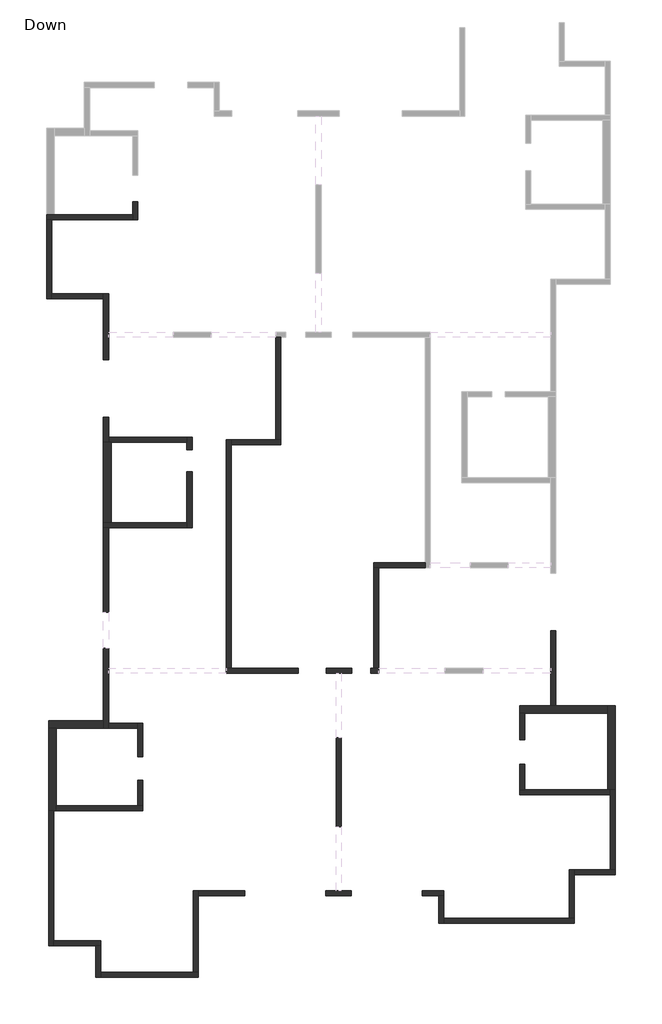
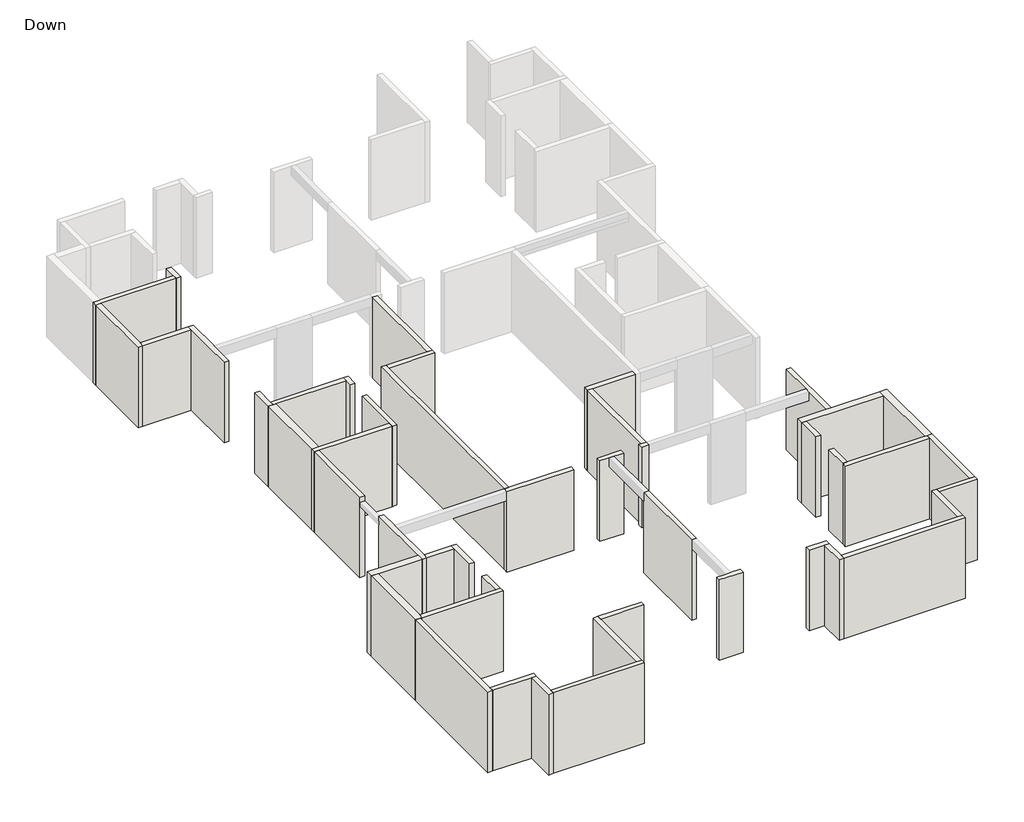
# One storey, part 1 of 2: 47 walls.
"""IFC4 building model written with IfcOpenShell, lengths in millimetres."""

from ifc_helpers import new_model, si_unit, origin, place, context, project, spatial, faceted_brep, element, save

model = new_model("IFC4")

# Units and contexts
model_context = context("Model", 3, world=origin())
ifc_project = project(units=[si_unit("LENGTHUNIT", "METRE", prefix="MILLI")], contexts=[model_context])

# Site, building, storey
site = spatial("IfcSite", under=ifc_project)
building = spatial("IfcBuilding", under=site)
storey = spatial("IfcBuildingStorey", under=building, Name="Down", Elevation=0.0)

# Walls
placement = place(None, origin())
element("IfcWall", 1, ObjectType="20", at=placement, inside=storey, context=model_context, shape_type="Brep", body=[
    faceted_brep([(-11352.0616697, 15349.6557961, 0.0), (-11352.0616697, 14832.6787416, 0.0), (-11352.0616697, 14632.6787416, 0.0), (-11352.0616697, 14632.6787416, 3600.0), (-11352.0616697, 14832.6787416, 3600.0), (-11352.0616697, 15349.6557961, 3600.0), (-11352.0616697, 15349.6557961, 3360.0), (-11152.0616697, 15349.6557961, 0.0), (-11152.0616697, 15349.6557961, 3360.0), (-11152.0616697, 15349.6557961, 3600.0), (-11152.0616697, 14632.6787416, 3600.0), (-11152.0616697, 14632.6787416, 3360.0), (-11152.0616697, 14632.6787416, 0.0)], [[[0, 1, 2, 3, 4, 5, 6]], [[7, 8, 9, 10, 11, 12]], [[2, 1, 0, 7, 12]], [[5, 4, 3, 10, 9]], [[0, 6, 5, 9, 8, 7]], [[3, 2, 12, 11, 10]]]),
])
element("IfcWall", 2, ObjectType="20", at=placement, inside=storey, context=model_context, shape_type="Brep", body=[
    faceted_brep([(-11352.0616697, 14832.6787416, 0.0), (-14451.9956956, 14832.6787416, 0.0), (-14752.0616697, 14832.6787416, 0.0), (-14752.0616697, 14832.6787416, 3600.0), (-14451.9956956, 14832.6787416, 3600.0), (-11352.0616697, 14832.6787416, 3600.0), (-11352.0616697, 14832.6787416, 3360.0), (-11352.0616697, 14632.6787416, 0.0), (-11352.0616697, 14632.6787416, 3600.0), (-14552.0616697, 14632.6787416, 3600.0), (-14752.0616697, 14632.6787416, 3600.0), (-14752.0616697, 14632.6787416, 0.0), (-14552.0616697, 14632.6787416, 0.0)], [[[0, 1, 2, 3, 4, 5, 6]], [[7, 8, 9, 10, 11, 12]], [[2, 1, 0, 7, 12, 11]], [[5, 4, 3, 10, 9, 8]], [[0, 6, 5, 8, 7]], [[3, 2, 11, 10]]]),
])
element("IfcWall", 3, ObjectType="20", at=placement, inside=storey, context=model_context, shape_type="Brep", body=[
    faceted_brep([(-14752.0616697, 14632.6787416, 0.0), (-14752.0616697, 11525.7761998, 0.0), (-14752.0616697, 11525.7761998, 3600.0), (-14752.0616697, 14632.6787416, 3600.0), (-14552.0616697, 14632.6787416, 0.0), (-14552.0616697, 14632.6787416, 3360.0), (-14552.0616697, 14632.6787416, 3600.0), (-14552.0616697, 11725.7761998, 3600.0), (-14552.0616697, 11525.7761998, 3600.0), (-14552.0616697, 11525.7761998, 0.0), (-14552.0616697, 11725.7761998, 0.0)], [[[0, 1, 2, 3]], [[4, 5, 6, 7, 8, 9, 10]], [[1, 0, 4, 10, 9]], [[3, 2, 8, 7, 6]], [[0, 3, 6, 5, 4]], [[2, 1, 9, 8]]]),
])
element("IfcWall", 4, ObjectType="20", at=placement, inside=storey, context=model_context, shape_type="Brep", body=[
    faceted_brep([(-14552.0616697, 11525.7761998, 0.0), (-12510.2559741, 11525.7761998, 0.0), (-12510.2559741, 11525.7761998, 3600.0), (-14552.0616697, 11525.7761998, 3600.0), (-14552.0616697, 11725.7761998, 0.0), (-14552.0616697, 11725.7761998, 3360.0), (-14552.0616697, 11725.7761998, 3600.0), (-12510.2559741, 11725.7761998, 3600.0), (-12510.2559741, 11725.7761998, 0.0)], [[[0, 1, 2, 3]], [[4, 5, 6, 7, 8]], [[1, 0, 4, 8]], [[3, 2, 7, 6]], [[0, 3, 6, 5, 4]], [[2, 1, 8, 7]]]),
])
element("IfcWall", 5, ObjectType="20", at=placement, inside=storey, context=model_context, shape_type="Brep", body=[
    faceted_brep([(-12510.2559741, 11725.7761998, 0.0), (-12510.2559741, 11525.7761998, 0.0), (-12510.2559741, 9117.4688625, 0.0), (-12510.2559741, 9117.4688625, 3360.0), (-12510.2559741, 9117.4688625, 3600.0), (-12510.2559741, 10265.7196834, 3600.0), (-12510.2559741, 11525.7761998, 3600.0), (-12510.2559741, 11725.7761998, 3600.0), (-12310.2559741, 11725.7761998, 0.0), (-12310.2559741, 11725.7761998, 3360.0), (-12310.2559741, 11725.7761998, 3600.0), (-12310.2559741, 10202.1270927, 3600.0), (-12310.2559741, 10002.1270927, 3600.0), (-12310.2559741, 9117.4688625, 3600.0), (-12310.2559741, 9117.4688625, 3360.0), (-12310.2559741, 9117.4688625, 0.0)], [[[0, 1, 2, 3, 4, 5, 6, 7]], [[8, 9, 10, 11, 12, 13, 14, 15]], [[2, 1, 0, 8, 15]], [[4, 3, 2, 15, 14, 13]], [[7, 6, 5, 4, 13, 12, 11, 10]], [[0, 7, 10, 9, 8]]]),
])
element("IfcWall", 6, ObjectType="20", at=placement, inside=storey, context=model_context, shape_type="Brep", body=[
    faceted_brep([(-12510.2559741, 6865.4241392, 0.0), (-12510.2559741, 5865.7196834, 0.0), (-12510.2559741, 5865.7196834, 3360.0), (-12510.2559741, 5865.7196834, 3600.0), (-12510.2559741, 6865.4241392, 3600.0), (-12510.2559741, 6865.4241392, 3360.0), (-12310.2559741, 6865.4241392, 0.0), (-12310.2559741, 6865.4241392, 3360.0), (-12310.2559741, 6865.4241392, 3600.0), (-12310.2559741, 6065.7196834, 3600.0), (-12310.2559741, 5865.7196834, 3600.0), (-12310.2559741, 5865.7196834, 0.0), (-12310.2559741, 6065.7196834, 0.0)], [[[0, 1, 2, 3, 4, 5]], [[6, 7, 8, 9, 10, 11, 12]], [[1, 0, 6, 12, 11]], [[4, 3, 10, 9, 8]], [[0, 5, 4, 8, 7, 6]], [[3, 2, 1, 11, 10]]]),
])
element("IfcWall", 7, ObjectType="20", at=placement, inside=storey, context=model_context, shape_type="Brep", body=[
    faceted_brep([(-12310.2559741, 5865.7196834, 0.0), (-12210.2559741, 5865.7196834, 0.0), (-9219.5123561, 5865.7196834, 0.0), (-9219.5123561, 5865.7196834, 3360.0), (-9219.5123561, 5865.7196834, 3600.0), (-12210.2559741, 5865.7196834, 3600.0), (-12310.2559741, 5865.7196834, 3600.0), (-12310.2559741, 6065.7196834, 0.0), (-12310.2559741, 6065.7196834, 3360.0), (-12310.2559741, 6065.7196834, 3600.0), (-9219.5123561, 6065.7196834, 3600.0), (-9219.5123561, 6065.7196834, 0.0)], [[[0, 1, 2, 3, 4, 5, 6]], [[7, 8, 9, 10, 11]], [[2, 1, 0, 7, 11]], [[6, 5, 4, 10, 9]], [[0, 6, 9, 8, 7]], [[4, 3, 2, 11, 10]]]),
])
element("IfcWall", 8, ObjectType="20", at=placement, inside=storey, context=model_context, shape_type="Brep", body=[
    faceted_brep([(-9219.5123561, 6065.7196834, 0.0), (-9219.5123561, 5865.7196834, 0.0), (-9219.5123561, 5569.3499325, 0.0), (-9219.5123561, 5569.3499325, 3360.0), (-9219.5123561, 5569.3499325, 3600.0), (-9219.5123561, 5865.7196834, 3600.0), (-9219.5123561, 6065.7196834, 3600.0), (-9019.5123561, 6065.7196834, 0.0), (-9019.5123561, 6065.7196834, 3360.0), (-9019.5123561, 6065.7196834, 3600.0), (-9019.5123561, 5569.3499325, 3600.0), (-9019.5123561, 5569.3499325, 3360.0), (-9019.5123561, 5569.3499325, 0.0)], [[[0, 1, 2, 3, 4, 5, 6]], [[7, 8, 9, 10, 11, 12]], [[2, 1, 0, 7, 12]], [[4, 3, 2, 12, 11, 10]], [[6, 5, 4, 10, 9]], [[0, 6, 9, 8, 7]]]),
])
element("IfcWall", 9, ObjectType="20", at=placement, inside=storey, context=model_context, shape_type="Brep", body=[
    faceted_brep([(-9219.5123561, 4705.2999252, 0.0), (-9219.5123561, 2708.4085645, 0.0), (-9219.5123561, 2508.4085645, 0.0), (-9219.5123561, 2508.4085645, 3600.0), (-9219.5123561, 2708.4085645, 3600.0), (-9219.5123561, 4705.2999252, 3600.0), (-9219.5123561, 4705.2999252, 3360.0), (-9019.5123561, 4705.2999252, 0.0), (-9019.5123561, 4705.2999252, 3360.0), (-9019.5123561, 4705.2999252, 3600.0), (-9019.5123561, 2508.4085645, 3600.0), (-9019.5123561, 2508.4085645, 3360.0), (-9019.5123561, 2508.4085645, 0.0)], [[[0, 1, 2, 3, 4, 5, 6]], [[7, 8, 9, 10, 11, 12]], [[2, 1, 0, 7, 12]], [[5, 4, 3, 10, 9]], [[0, 6, 5, 9, 8, 7]], [[3, 2, 12, 11, 10]]]),
])
element("IfcWall", 10, ObjectType="20", at=placement, inside=storey, context=model_context, shape_type="Brep", body=[
    faceted_brep([(-9219.5123561, 2708.4085645, 0.0), (-12210.2559741, 2708.4085645, 0.0), (-12510.2559741, 2708.4085645, 0.0), (-12510.2559741, 2708.4085645, 3600.0), (-12210.2559741, 2708.4085645, 3600.0), (-9219.5123561, 2708.4085645, 3600.0), (-9219.5123561, 2708.4085645, 3360.0), (-9219.5123561, 2508.4085645, 0.0), (-9219.5123561, 2508.4085645, 3600.0), (-12310.2559741, 2508.4085645, 3600.0), (-12510.2559741, 2508.4085645, 3600.0), (-12510.2559741, 2508.4085645, 0.0), (-12310.2559741, 2508.4085645, 0.0)], [[[0, 1, 2, 3, 4, 5, 6]], [[7, 8, 9, 10, 11, 12]], [[2, 1, 0, 7, 12, 11]], [[5, 4, 3, 10, 9, 8]], [[0, 6, 5, 8, 7]], [[3, 2, 11, 10]]]),
])
element("IfcWall", 11, ObjectType="20", at=placement, inside=storey, context=model_context, shape_type="Brep", body=[
    faceted_brep([(-12510.2559741, 2508.4085645, 0.0), (-12510.2559741, -828.2926655, 0.0), (-12510.2559741, -828.2926655, 3200.0), (-12510.2559741, -828.2926655, 3360.0), (-12510.2559741, -828.2926655, 3600.0), (-12510.2559741, 2508.4085645, 3600.0), (-12310.2559741, 2508.4085645, 0.0), (-12310.2559741, 2508.4085645, 3360.0), (-12310.2559741, 2508.4085645, 3600.0), (-12310.2559741, -828.2926655, 3600.0), (-12310.2559741, -828.2926655, 3360.0), (-12310.2559741, -828.2926655, 3200.0), (-12310.2559741, -828.2926655, 0.0)], [[[0, 1, 2, 3, 4, 5]], [[6, 7, 8, 9, 10, 11, 12]], [[1, 0, 6, 12]], [[4, 3, 2, 1, 12, 11, 10, 9]], [[5, 4, 9, 8]], [[0, 5, 8, 7, 6]]]),
])
element("IfcWall", 12, ObjectType="20", at=placement, inside=storey, context=model_context, shape_type="Brep", body=[
    faceted_brep([(-12510.2559741, -2234.6718166, 0.0), (-12510.2559741, -5102.5799771, 0.0), (-12510.2559741, -5402.5799771, 0.0), (-12510.2559741, -5402.5799771, 3600.0), (-12510.2559741, -5102.5799771, 3600.0), (-12510.2559741, -2234.6718166, 3600.0), (-12510.2559741, -2234.6718166, 3360.0), (-12510.2559741, -2234.6718166, 3200.0), (-12310.2559741, -2234.6718166, 0.0), (-12310.2559741, -2234.6718166, 3200.0), (-12310.2559741, -2234.6718166, 3360.0), (-12310.2559741, -2234.6718166, 3600.0), (-12310.2559741, -3027.4112609, 3600.0), (-12310.2559741, -3227.4112609, 3600.0), (-12310.2559741, -5203.6927327, 3600.0), (-12310.2559741, -5402.5799771, 3600.0), (-12310.2559741, -5402.5799771, 3360.0), (-12310.2559741, -5402.5799771, 0.0), (-12310.2559741, -5203.6927327, 0.0)], [[[0, 1, 2, 3, 4, 5, 6, 7]], [[8, 9, 10, 11, 12, 13, 14, 15, 16, 17, 18]], [[2, 1, 0, 8, 18, 17]], [[5, 4, 3, 15, 14, 13, 12, 11]], [[0, 7, 6, 5, 11, 10, 9, 8]], [[3, 2, 17, 16, 15]]]),
])
element("IfcWall", 13, ObjectType="20", at=placement, inside=storey, context=model_context, shape_type="Brep", body=[
    faceted_brep([(-14372.6039184, -8641.5084419, 0.0), (-10959.0284047, -8641.5084419, 0.0), (-10959.0284047, -8641.5084419, 3360.0), (-10959.0284047, -8641.5084419, 3600.0), (-14372.6039184, -8641.5084419, 3600.0), (-14372.6039184, -8441.5084419, 0.0), (-14372.6039184, -8441.5084419, 3360.0), (-14372.6039184, -8441.5084419, 3600.0), (-11159.0284047, -8441.5084419, 3600.0), (-10959.0284047, -8441.5084419, 3600.0), (-10959.0284047, -8441.5084419, 0.0), (-11159.0284047, -8441.5084419, 0.0)], [[[0, 1, 2, 3, 4]], [[5, 6, 7, 8, 9, 10, 11]], [[1, 0, 5, 11, 10]], [[4, 3, 9, 8, 7]], [[3, 2, 1, 10, 9]], [[0, 4, 7, 6, 5]]]),
])
element("IfcWall", 14, ObjectType="20", at=placement, inside=storey, context=model_context, shape_type="Brep", body=[
    faceted_brep([(-10959.0284047, -8441.5084419, 0.0), (-10959.0284047, -7441.5084419, 0.0), (-10959.0284047, -7441.5084419, 3360.0), (-10959.0284047, -7441.5084419, 3600.0), (-10959.0284047, -8441.5084419, 3600.0), (-11159.0284047, -8441.5084419, 0.0), (-11159.0284047, -8441.5084419, 3360.0), (-11159.0284047, -8441.5084419, 3600.0), (-11159.0284047, -7441.5084419, 3600.0), (-11159.0284047, -7441.5084419, 3360.0), (-11159.0284047, -7441.5084419, 0.0)], [[[0, 1, 2, 3, 4]], [[5, 6, 7, 8, 9, 10]], [[1, 0, 5, 10]], [[3, 2, 1, 10, 9, 8]], [[4, 3, 8, 7]], [[0, 4, 7, 6, 5]]]),
])
element("IfcWall", 15, ObjectType="20", at=placement, inside=storey, context=model_context, shape_type="Brep", body=[
    faceted_brep([(-10959.0284047, -6518.1513745, 0.0), (-10959.0284047, -5203.6927327, 0.0), (-10959.0284047, -5203.6927327, 3360.0), (-10959.0284047, -5203.6927327, 3600.0), (-10959.0284047, -6518.1513745, 3600.0), (-10959.0284047, -6518.1513745, 3360.0), (-11159.0284047, -6518.1513745, 0.0), (-11159.0284047, -6518.1513745, 3360.0), (-11159.0284047, -6518.1513745, 3600.0), (-11159.0284047, -5403.6927327, 3600.0), (-11159.0284047, -5203.6927327, 3600.0), (-11159.0284047, -5203.6927327, 0.0), (-11159.0284047, -5403.6927327, 0.0)], [[[0, 1, 2, 3, 4, 5]], [[6, 7, 8, 9, 10, 11, 12]], [[1, 0, 6, 12, 11]], [[4, 3, 10, 9, 8]], [[0, 5, 4, 8, 7, 6]], [[3, 2, 1, 11, 10]]]),
])
element("IfcWall", 16, ObjectType="20", at=placement, inside=storey, context=model_context, shape_type="Brep", body=[
    faceted_brep([(-11159.0284047, -5203.6927327, 0.0), (-12310.2559741, -5203.6927327, 0.0), (-12310.2559741, -5203.6927327, 3360.0), (-12310.2559741, -5203.6927327, 3600.0), (-11159.0284047, -5203.6927327, 3600.0), (-11159.0284047, -5403.6927327, 0.0), (-11159.0284047, -5403.6927327, 3360.0), (-11159.0284047, -5403.6927327, 3600.0), (-12310.2559741, -5403.6927327, 3600.0), (-12310.2559741, -5403.6927327, 3360.0), (-12310.2559741, -5403.6927327, 0.0), (-12310.2559741, -5402.5799771, 0.0), (-12310.2559741, -5402.5799771, 3600.0)], [[[0, 1, 2, 3, 4]], [[5, 6, 7, 8, 9, 10]], [[1, 0, 5, 10, 11]], [[4, 3, 12, 8, 7]], [[0, 4, 7, 6, 5]], [[3, 2, 1, 11, 10, 9, 8, 12]]]),
])
element("IfcWall", 17, ObjectType="20", at=placement, inside=storey, context=model_context, shape_type="Brep", body=[
    faceted_brep([(-14672.6039184, -8641.5084419, 0.0), (-14672.6039184, -13963.683275, 0.0), (-14672.6039184, -13963.683275, 3600.0), (-14672.6039184, -8641.5084419, 3600.0), (-14472.6039184, -8641.5084419, 0.0), (-14472.6039184, -8641.5084419, 3360.0), (-14472.6039184, -8641.5084419, 3600.0), (-14472.6039184, -13763.683275, 3600.0), (-14472.6039184, -13963.683275, 3600.0), (-14472.6039184, -13963.683275, 0.0), (-14472.6039184, -13763.683275, 0.0)], [[[0, 1, 2, 3]], [[4, 5, 6, 7, 8, 9, 10]], [[1, 0, 4, 10, 9]], [[3, 2, 8, 7, 6]], [[2, 1, 9, 8]], [[0, 3, 6, 5, 4]]]),
])
element("IfcWall", 18, ObjectType="20", at=placement, inside=storey, context=model_context, shape_type="Brep", body=[
    faceted_brep([(-14472.6039184, -13963.683275, 0.0), (-12822.7829253, -13963.683275, 0.0), (-12622.7829253, -13963.683275, 0.0), (-12622.7829253, -13963.683275, 3600.0), (-12822.7829253, -13963.683275, 3600.0), (-14472.6039184, -13963.683275, 3600.0), (-14472.6039184, -13763.683275, 0.0), (-14472.6039184, -13763.683275, 3360.0), (-14472.6039184, -13763.683275, 3600.0), (-12622.7829253, -13763.683275, 3600.0), (-12622.7829253, -13763.683275, 3360.0), (-12622.7829253, -13763.683275, 0.0)], [[[0, 1, 2, 3, 4, 5]], [[6, 7, 8, 9, 10, 11]], [[2, 1, 0, 6, 11]], [[5, 4, 3, 9, 8]], [[0, 5, 8, 7, 6]], [[3, 2, 11, 10, 9]]]),
])
element("IfcWall", 19, ObjectType="20", at=placement, inside=storey, context=model_context, shape_type="Brep", body=[
    faceted_brep([(-12822.7829253, -13963.683275, 0.0), (-12822.7829253, -15213.7980888, 0.0), (-12822.7829253, -15213.7980888, 3600.0), (-12822.7829253, -13963.683275, 3600.0), (-12622.7829253, -13963.683275, 0.0), (-12622.7829253, -13963.683275, 3600.0), (-12622.7829253, -15013.7980888, 3600.0), (-12622.7829253, -15213.7980888, 3600.0), (-12622.7829253, -15213.7980888, 0.0), (-12622.7829253, -15013.7980888, 0.0)], [[[0, 1, 2, 3]], [[4, 5, 6, 7, 8, 9]], [[1, 0, 4, 9, 8]], [[3, 2, 7, 6, 5]], [[0, 3, 5, 4]], [[2, 1, 8, 7]]]),
])
element("IfcWall", 20, ObjectType="20", at=placement, inside=storey, context=model_context, shape_type="Brep", body=[
    faceted_brep([(-12622.7829253, -15213.7980888, 0.0), (-8771.3292903, -15213.7980888, 0.0), (-8771.3292903, -15213.7980888, 3600.0), (-12622.7829253, -15213.7980888, 3600.0), (-12622.7829253, -15013.7980888, 0.0), (-12622.7829253, -15013.7980888, 3360.0), (-12622.7829253, -15013.7980888, 3600.0), (-8971.3292903, -15013.7980888, 3600.0), (-8771.3292903, -15013.7980888, 3600.0), (-8771.3292903, -15013.7980888, 0.0), (-8971.3292903, -15013.7980888, 0.0)], [[[0, 1, 2, 3]], [[4, 5, 6, 7, 8, 9, 10]], [[1, 0, 4, 10, 9]], [[3, 2, 8, 7, 6]], [[0, 3, 6, 5, 4]], [[2, 1, 9, 8]]]),
])
element("IfcWall", 21, ObjectType="20", at=placement, inside=storey, context=model_context, shape_type="Brep", body=[
    faceted_brep([(-8771.3292903, -15013.7980888, 0.0), (-8771.3292903, -11996.592326, 0.0), (-8771.3292903, -11796.592326, 0.0), (-8771.3292903, -11796.592326, 3600.0), (-8771.3292903, -11996.592326, 3600.0), (-8771.3292903, -14392.0600908, 3600.0), (-8771.3292903, -15013.7980888, 3600.0), (-8971.3292903, -15013.7980888, 0.0), (-8971.3292903, -15013.7980888, 3360.0), (-8971.3292903, -15013.7980888, 3600.0), (-8971.3292903, -11796.592326, 3600.0), (-8971.3292903, -11796.592326, 3360.0), (-8971.3292903, -11796.592326, 0.0)], [[[0, 1, 2, 3, 4, 5, 6]], [[7, 8, 9, 10, 11, 12]], [[2, 1, 0, 7, 12]], [[6, 5, 4, 3, 10, 9]], [[0, 6, 9, 8, 7]], [[3, 2, 12, 11, 10]]]),
])
element("IfcWall", 22, ObjectType="20", at=placement, inside=storey, context=model_context, shape_type="Brep", body=[
    faceted_brep([(-8771.3292903, -11996.592326, 0.0), (-6942.1181861, -11996.592326, 0.0), (-6942.1181861, -11996.592326, 3360.0), (-6942.1181861, -11996.592326, 3600.0), (-8771.3292903, -11996.592326, 3600.0), (-8771.3292903, -11996.592326, 3360.0), (-8771.3292903, -11796.592326, 0.0), (-8771.3292903, -11796.592326, 3600.0), (-6942.1181861, -11796.592326, 3600.0), (-6942.1181861, -11796.592326, 3360.0), (-6942.1181861, -11796.592326, 0.0)], [[[0, 1, 2, 3, 4, 5]], [[6, 7, 8, 9, 10]], [[1, 0, 6, 10]], [[3, 2, 1, 10, 9, 8]], [[4, 3, 8, 7]], [[0, 5, 4, 7, 6]]]),
])
element("IfcWall", 23, ObjectType="20", at=placement, inside=storey, context=model_context, shape_type="Brep", body=[
    faceted_brep([(-3743.2951349, -11996.592326, 0.0), (-2741.3652253, -11996.592326, 0.0), (-2741.3652253, -11996.592326, 3360.0), (-2741.3652253, -11996.592326, 3600.0), (-3743.2951349, -11996.592326, 3600.0), (-3743.2951349, -11996.592326, 3360.0), (-3743.2951349, -11796.592326, 0.0), (-3743.2951349, -11796.592326, 3360.0), (-3743.2951349, -11796.592326, 3600.0), (-3345.8144093, -11796.592326, 3600.0), (-3145.8144093, -11796.592326, 3600.0), (-2741.3652253, -11796.592326, 3600.0), (-2741.3652253, -11796.592326, 3360.0), (-2741.3652253, -11796.592326, 0.0)], [[[0, 1, 2, 3, 4, 5]], [[6, 7, 8, 9, 10, 11, 12, 13]], [[1, 0, 6, 13]], [[3, 2, 1, 13, 12, 11]], [[4, 3, 11, 10, 9, 8]], [[0, 5, 4, 8, 7, 6]]]),
])
element("IfcWall", 24, ObjectType="20", at=placement, inside=storey, context=model_context, shape_type="Brep", body=[
    faceted_brep([(53.0069184, -11996.592326, 0.0), (698.6742141, -11996.592326, 0.0), (898.6742141, -11996.592326, 0.0), (898.6742141, -11996.592326, 3600.0), (698.6742141, -11996.592326, 3600.0), (53.0069184, -11996.592326, 3600.0), (53.0069184, -11996.592326, 3360.0), (53.0069184, -11796.592326, 0.0), (53.0069184, -11796.592326, 3360.0), (53.0069184, -11796.592326, 3600.0), (898.6742141, -11796.592326, 3600.0), (898.6742141, -11796.592326, 3360.0), (898.6742141, -11796.592326, 0.0)], [[[0, 1, 2, 3, 4, 5, 6]], [[7, 8, 9, 10, 11, 12]], [[2, 1, 0, 7, 12]], [[5, 4, 3, 10, 9]], [[0, 6, 5, 9, 8, 7]], [[3, 2, 12, 11, 10]]]),
])
element("IfcWall", 25, ObjectType="20", at=placement, inside=storey, context=model_context, shape_type="Brep", body=[
    faceted_brep([(698.6742141, -11996.592326, 0.0), (698.6742141, -13072.0600908, 0.0), (698.6742141, -13072.0600908, 3360.0), (698.6742141, -13072.0600908, 3600.0), (698.6742141, -11996.592326, 3600.0), (698.6742141, -11996.592326, 3360.0), (898.6742141, -11996.592326, 0.0), (898.6742141, -11996.592326, 3600.0), (898.6742141, -12872.0600908, 3600.0), (898.6742141, -13072.0600908, 3600.0), (898.6742141, -13072.0600908, 0.0), (898.6742141, -12872.0600908, 0.0)], [[[0, 1, 2, 3, 4, 5]], [[6, 7, 8, 9, 10, 11]], [[1, 0, 6, 11, 10]], [[4, 3, 9, 8, 7]], [[0, 5, 4, 7, 6]], [[3, 2, 1, 10, 9]]]),
])
element("IfcWall", 26, ObjectType="20", at=placement, inside=storey, context=model_context, shape_type="Brep", body=[
    faceted_brep([(898.6742141, -13072.0600908, 0.0), (6046.2020558, -13072.0600908, 0.0), (6046.2020558, -13072.0600908, 3600.0), (3446.2020558, -13072.0600908, 3600.0), (898.6742141, -13072.0600908, 3600.0), (898.6742141, -12872.0600908, 0.0), (898.6742141, -12872.0600908, 3360.0), (898.6742141, -12872.0600908, 3600.0), (5846.2020558, -12872.0600908, 3600.0), (6046.2020558, -12872.0600908, 3600.0), (6046.2020558, -12872.0600908, 0.0), (5846.2020558, -12872.0600908, 0.0)], [[[0, 1, 2, 3, 4]], [[5, 6, 7, 8, 9, 10, 11]], [[1, 0, 5, 11, 10]], [[4, 3, 2, 9, 8, 7]], [[0, 4, 7, 6, 5]], [[2, 1, 10, 9]]]),
])
element("IfcWall", 27, ObjectType="20", at=placement, inside=storey, context=model_context, shape_type="Brep", body=[
    faceted_brep([(6046.2020558, -12872.0600908, 0.0), (6046.2020558, -11167.0874585, 0.0), (6046.2020558, -10967.0874585, 0.0), (6046.2020558, -10967.0874585, 3600.0), (6046.2020558, -11167.0874585, 3600.0), (6046.2020558, -12872.0600908, 3600.0), (5846.2020558, -12872.0600908, 0.0), (5846.2020558, -12872.0600908, 3360.0), (5846.2020558, -12872.0600908, 3600.0), (5846.2020558, -10967.0874585, 3600.0), (5846.2020558, -10967.0874585, 3360.0), (5846.2020558, -10967.0874585, 0.0)], [[[0, 1, 2, 3, 4, 5]], [[6, 7, 8, 9, 10, 11]], [[2, 1, 0, 6, 11]], [[5, 4, 3, 9, 8]], [[0, 5, 8, 7, 6]], [[3, 2, 11, 10, 9]]]),
])
element("IfcWall", 28, ObjectType="20", at=placement, inside=storey, context=model_context, shape_type="Brep", body=[
    faceted_brep([(6046.2020558, -11167.0874585, 0.0), (7654.8049372, -11167.0874585, 0.0), (7654.8049372, -11167.0874585, 3600.0), (6046.2020558, -11167.0874585, 3600.0), (6046.2020558, -10967.0874585, 0.0), (6046.2020558, -10967.0874585, 3600.0), (7454.8049372, -10967.0874585, 3600.0), (7654.8049372, -10967.0874585, 3600.0), (7654.8049372, -10967.0874585, 0.0), (7454.8049372, -10967.0874585, 0.0)], [[[0, 1, 2, 3]], [[4, 5, 6, 7, 8, 9]], [[1, 0, 4, 9, 8]], [[3, 2, 7, 6, 5]], [[0, 3, 5, 4]], [[2, 1, 8, 7]]]),
])
element("IfcWall", 29, ObjectType="20", at=placement, inside=storey, context=model_context, shape_type="Brep", body=[
    faceted_brep([(7654.8049372, -10967.0874585, 0.0), (7654.8049372, -7816.451035, 0.0), (7654.8049372, -7816.451035, 3600.0), (7654.8049372, -10967.0874585, 3600.0), (7454.8049372, -10967.0874585, 0.0), (7454.8049372, -10967.0874585, 3360.0), (7454.8049372, -10967.0874585, 3600.0), (7454.8049372, -8016.451035, 3600.0), (7454.8049372, -7816.451035, 3600.0), (7454.8049372, -7816.451035, 0.0), (7454.8049372, -8016.451035, 0.0)], [[[0, 1, 2, 3]], [[4, 5, 6, 7, 8, 9, 10]], [[1, 0, 4, 10, 9]], [[3, 2, 8, 7, 6]], [[0, 3, 6, 5, 4]], [[2, 1, 9, 8]]]),
])
element("IfcWall", 30, ObjectType="20", at=placement, inside=storey, context=model_context, shape_type="Brep", body=[
    faceted_brep([(3886.0795653, -8016.451035, 0.0), (7454.8049372, -8016.451035, 0.0), (7454.8049372, -8016.451035, 3360.0), (7454.8049372, -8016.451035, 3600.0), (3886.0795653, -8016.451035, 3600.0), (3886.0795653, -8016.451035, 3360.0), (3886.0795653, -7816.451035, 0.0), (3886.0795653, -7816.451035, 3600.0), (4086.0795653, -7816.451035, 3600.0), (7354.8049372, -7816.451035, 3600.0), (7454.8049372, -7816.451035, 3600.0), (7454.8049372, -7816.451035, 0.0), (7354.8049372, -7816.451035, 0.0), (4086.0795653, -7816.451035, 0.0)], [[[0, 1, 2, 3, 4, 5]], [[6, 7, 8, 9, 10, 11, 12, 13]], [[1, 0, 6, 13, 12, 11]], [[4, 3, 10, 9, 8, 7]], [[3, 2, 1, 11, 10]], [[0, 5, 4, 7, 6]]]),
])
element("IfcWall", 31, ObjectType="20", at=placement, inside=storey, context=model_context, shape_type="Brep", body=[
    faceted_brep([(3886.0795653, -4814.2914978, 0.0), (3886.0795653, -5856.32504, 0.0), (3886.0795653, -5856.32504, 3360.0), (3886.0795653, -5856.32504, 3600.0), (3886.0795653, -4814.2914978, 3600.0), (4086.0795653, -4814.2914978, 0.0), (4086.0795653, -4814.2914978, 3360.0), (4086.0795653, -4814.2914978, 3600.0), (4086.0795653, -5856.32504, 3600.0), (4086.0795653, -5856.32504, 3360.0), (4086.0795653, -5856.32504, 0.0)], [[[0, 1, 2, 3, 4]], [[5, 6, 7, 8, 9, 10]], [[1, 0, 5, 10]], [[3, 2, 1, 10, 9, 8]], [[4, 3, 8, 7]], [[0, 4, 7, 6, 5]]]),
])
element("IfcWall", 32, ObjectType="20", at=placement, inside=storey, context=model_context, shape_type="Brep", body=[
    faceted_brep([(3886.0795653, -6812.2956141, 0.0), (3886.0795653, -7816.451035, 0.0), (3886.0795653, -7816.451035, 3600.0), (3886.0795653, -6812.2956141, 3600.0), (3886.0795653, -6812.2956141, 3360.0), (4086.0795653, -6812.2956141, 0.0), (4086.0795653, -6812.2956141, 3360.0), (4086.0795653, -6812.2956141, 3600.0), (4086.0795653, -7816.451035, 3600.0), (4086.0795653, -7816.451035, 3360.0), (4086.0795653, -7816.451035, 0.0)], [[[0, 1, 2, 3, 4]], [[5, 6, 7, 8, 9, 10]], [[1, 0, 5, 10]], [[3, 2, 8, 7]], [[0, 4, 3, 7, 6, 5]], [[2, 1, 10, 9, 8]]]),
])
element("IfcWall", 33, ObjectType="20", at=placement, inside=storey, context=model_context, shape_type="Brep", body=[
    faceted_brep([(5308.6159742, -4514.2914978, 0.0), (5308.6159742, -1563.6550168, 0.0), (5308.6159742, -1563.6550168, 3360.0), (5308.6159742, -1563.6550168, 3600.0), (5308.6159742, -4514.2914978, 3600.0), (5308.6159742, -4514.2914978, 3360.0), (5108.6159742, -4514.2914978, 0.0), (5108.6159742, -4514.2914978, 3360.0), (5108.6159742, -4514.2914978, 3600.0), (5108.6159742, -3227.4112609, 3600.0), (5108.6159742, -3027.4112609, 3600.0), (5108.6159742, -1563.6550168, 3600.0), (5108.6159742, -1563.6550168, 3360.0), (5108.6159742, -1563.6550168, 0.0)], [[[0, 1, 2, 3, 4, 5]], [[6, 7, 8, 9, 10, 11, 12, 13]], [[1, 0, 6, 13]], [[3, 2, 1, 13, 12, 11]], [[4, 3, 11, 10, 9, 8]], [[0, 5, 4, 8, 7, 6]]]),
])
element("IfcWall", 34, ObjectType="20", at=placement, inside=storey, context=model_context, shape_type="Brep", body=[
    faceted_brep([(-7668.2865676, -3227.4112609, 0.0), (-4837.1456113, -3227.4112609, 0.0), (-4837.1456113, -3227.4112609, 3360.0), (-4837.1456113, -3227.4112609, 3600.0), (-7668.2865676, -3227.4112609, 3600.0), (-7668.2865676, -3227.4112609, 3200.0), (-7668.2865676, -3027.4112609, 0.0), (-7668.2865676, -3027.4112609, 3200.0), (-7668.2865676, -3027.4112609, 3600.0), (-7468.2865676, -3027.4112609, 3600.0), (-4837.1456113, -3027.4112609, 3600.0), (-4837.1456113, -3027.4112609, 3360.0), (-4837.1456113, -3027.4112609, 0.0), (-7468.2865676, -3027.4112609, 0.0)], [[[0, 1, 2, 3, 4, 5]], [[6, 7, 8, 9, 10, 11, 12, 13]], [[1, 0, 6, 13, 12]], [[3, 2, 1, 12, 11, 10]], [[4, 3, 10, 9, 8]], [[0, 5, 4, 8, 7, 6]]]),
])
element("IfcWall", 35, ObjectType="20", at=placement, inside=storey, context=model_context, shape_type="Brep", body=[
    faceted_brep([(-7468.2865676, -3027.4112609, 0.0), (-7468.2865676, 5773.799174, 0.0), (-7468.2865676, 5973.799174, 0.0), (-7468.2865676, 5973.799174, 3600.0), (-7468.2865676, 5773.799174, 3600.0), (-7468.2865676, -3027.4112609, 3600.0), (-7668.2865676, -3027.4112609, 0.0), (-7668.2865676, -3027.4112609, 3360.0), (-7668.2865676, -3027.4112609, 3600.0), (-7668.2865676, 5973.799174, 3600.0), (-7668.2865676, 5973.799174, 3360.0), (-7668.2865676, 5973.799174, 0.0)], [[[0, 1, 2, 3, 4, 5]], [[6, 7, 8, 9, 10, 11]], [[2, 1, 0, 6, 11]], [[5, 4, 3, 9, 8]], [[0, 5, 8, 7, 6]], [[3, 2, 11, 10, 9]]]),
])
element("IfcWall", 36, ObjectType="20", at=placement, inside=storey, context=model_context, shape_type="Brep", body=[
    faceted_brep([(-7468.2865676, 5773.799174, 0.0), (-5526.5468462, 5773.799174, 0.0), (-5526.5468462, 5773.799174, 3600.0), (-7468.2865676, 5773.799174, 3600.0), (-7468.2865676, 5973.799174, 0.0), (-7468.2865676, 5973.799174, 3600.0), (-5726.5468462, 5973.799174, 3600.0), (-5526.5468462, 5973.799174, 3600.0), (-5526.5468462, 5973.799174, 0.0), (-5726.5468462, 5973.799174, 0.0)], [[[0, 1, 2, 3]], [[4, 5, 6, 7, 8, 9]], [[1, 0, 4, 9, 8]], [[3, 2, 7, 6, 5]], [[0, 3, 5, 4]], [[2, 1, 8, 7]]]),
])
element("IfcWall", 37, ObjectType="20", at=placement, inside=storey, context=model_context, shape_type="Brep", body=[
    faceted_brep([(-5526.5468462, 5973.799174, 0.0), (-5526.5468462, 10002.1270927, 0.0), (-5526.5468462, 10002.1270927, 3600.0), (-5526.5468462, 5973.799174, 3600.0), (-5726.5468462, 5973.799174, 0.0), (-5726.5468462, 5973.799174, 3360.0), (-5726.5468462, 5973.799174, 3600.0), (-5726.5468462, 10002.1270927, 3600.0), (-5726.5468462, 10002.1270927, 3360.0), (-5726.5468462, 10002.1270927, 0.0)], [[[0, 1, 2, 3]], [[4, 5, 6, 7, 8, 9]], [[1, 0, 4, 9]], [[3, 2, 7, 6]], [[0, 3, 6, 5, 4]], [[2, 1, 9, 8, 7]]]),
])
element("IfcWall", 38, ObjectType="20", at=placement, inside=storey, context=model_context, shape_type="Brep", body=[
    faceted_brep([(165.5355931, 1118.1901182, 0.0), (-1868.1246952, 1118.1901182, 0.0), (-1868.1246952, 1118.1901182, 3600.0), (165.5355931, 1118.1901182, 3600.0), (165.5355931, 918.1901182, 0.0), (165.5355931, 918.1901182, 3600.0), (-1668.1246952, 918.1901182, 3600.0), (-1868.1246952, 918.1901182, 3600.0), (-1868.1246952, 918.1901182, 0.0), (-1668.1246952, 918.1901182, 0.0)], [[[0, 1, 2, 3]], [[4, 5, 6, 7, 8, 9]], [[1, 0, 4, 9, 8]], [[3, 2, 7, 6, 5]], [[0, 3, 5, 4]], [[2, 1, 8, 7]]]),
])
element("IfcWall", 39, ObjectType="20", at=placement, inside=storey, context=model_context, shape_type="Brep", body=[
    faceted_brep([(-1868.1246952, 918.1901182, 0.0), (-1868.1246952, -3027.4112609, 0.0), (-1868.1246952, -3027.4112609, 3600.0), (-1868.1246952, 918.1901182, 3600.0), (-1668.1246952, 918.1901182, 0.0), (-1668.1246952, 918.1901182, 3360.0), (-1668.1246952, 918.1901182, 3600.0), (-1668.1246952, -3027.4112609, 3600.0), (-1668.1246952, -3027.4112609, 3360.0), (-1668.1246952, -3027.4112609, 0.0)], [[[0, 1, 2, 3]], [[4, 5, 6, 7, 8, 9]], [[1, 0, 4, 9]], [[3, 2, 7, 6]], [[0, 3, 6, 5, 4]], [[2, 1, 9, 8, 7]]]),
])
element("IfcWall", 40, ObjectType="20", at=placement, inside=storey, context=model_context, shape_type="Brep", body=[
    faceted_brep([(-1668.1246952, -3027.4112609, 0.0), (-1868.1246952, -3027.4112609, 0.0), (-1969.2374508, -3027.4112609, 0.0), (-1969.2374508, -3027.4112609, 3360.0), (-1969.2374508, -3027.4112609, 3600.0), (-1868.1246952, -3027.4112609, 3600.0), (-1668.1246952, -3027.4112609, 3600.0), (-1668.1246952, -3027.4112609, 3200.0), (-1668.1246952, -3227.4112609, 0.0), (-1668.1246952, -3227.4112609, 3200.0), (-1668.1246952, -3227.4112609, 3600.0), (-1969.2374508, -3227.4112609, 3600.0), (-1969.2374508, -3227.4112609, 3360.0), (-1969.2374508, -3227.4112609, 0.0)], [[[0, 1, 2, 3, 4, 5, 6, 7]], [[8, 9, 10, 11, 12, 13]], [[2, 1, 0, 8, 13]], [[4, 3, 2, 13, 12, 11]], [[6, 5, 4, 11, 10]], [[0, 7, 6, 10, 9, 8]]]),
])
element("IfcWall", 41, ObjectType="20", at=placement, inside=storey, context=model_context, shape_type="Brep", body=[
    faceted_brep([(-2732.1747025, -3027.4112609, 0.0), (-3734.1028886, -3027.4112609, 0.0), (-3734.1028886, -3027.4112609, 3360.0), (-3734.1028886, -3027.4112609, 3600.0), (-2732.1747025, -3027.4112609, 3600.0), (-2732.1747025, -3027.4112609, 3360.0), (-2732.1747025, -3227.4112609, 0.0), (-2732.1747025, -3227.4112609, 3360.0), (-2732.1747025, -3227.4112609, 3600.0), (-3145.8144093, -3227.4112609, 3600.0), (-3345.8144093, -3227.4112609, 3600.0), (-3734.1028886, -3227.4112609, 3600.0), (-3734.1028886, -3227.4112609, 3360.0), (-3734.1028886, -3227.4112609, 0.0)], [[[0, 1, 2, 3, 4, 5]], [[6, 7, 8, 9, 10, 11, 12, 13]], [[1, 0, 6, 13]], [[3, 2, 1, 13, 12, 11]], [[4, 3, 11, 10, 9, 8]], [[0, 5, 4, 8, 7, 6]]]),
])
element("IfcWall", 42, ObjectType="20", at=placement, inside=storey, context=model_context, shape_type="Brep", body=[
    faceted_brep([(-3145.8144093, -9275.756314, 0.0), (-3145.8144093, -5775.756314, 0.0), (-3145.8144093, -5775.756314, 3200.0), (-3145.8144093, -5775.756314, 3600.0), (-3145.8144093, -9275.756314, 3600.0), (-3145.8144093, -9275.756314, 3200.0), (-3345.8144093, -9275.756314, 0.0), (-3345.8144093, -9275.756314, 3200.0), (-3345.8144093, -9275.756314, 3600.0), (-3345.8144093, -5775.756314, 3600.0), (-3345.8144093, -5775.756314, 3200.0), (-3345.8144093, -5775.756314, 0.0)], [[[0, 1, 2, 3, 4, 5]], [[6, 7, 8, 9, 10, 11]], [[1, 0, 6, 11]], [[3, 2, 1, 11, 10, 9]], [[4, 3, 9, 8]], [[0, 5, 4, 8, 7, 6]]]),
])
element("IfcWall", 43, ObjectType="30", at=placement, inside=storey, context=model_context, shape_type="Brep", body=[
    faceted_brep([(-12510.2559741, 5865.7196834, 0.0), (-12510.2559741, 2708.4085645, 0.0), (-12510.2559741, 2708.4085645, 3600.0), (-12510.2559741, 5865.7196834, 3600.0), (-12210.2559741, 5865.7196834, 0.0), (-12210.2559741, 5865.7196834, 3360.0), (-12210.2559741, 5865.7196834, 3600.0), (-12210.2559741, 2708.4085645, 3600.0), (-12210.2559741, 2708.4085645, 3360.0), (-12210.2559741, 2708.4085645, 0.0), (-12310.2559741, 5865.7196834, 0.0), (-12310.2559741, 5865.7196834, 3600.0)], [[[0, 1, 2, 3]], [[4, 5, 6, 7, 8, 9]], [[1, 0, 10, 4, 9]], [[3, 2, 7, 6, 11]], [[0, 3, 11, 6, 5, 4, 10]], [[2, 1, 9, 8, 7]]]),
])
element("IfcWall", 44, ObjectType="30", at=placement, inside=storey, context=model_context, shape_type="Brep", body=[
    faceted_brep([(-14672.6039184, -5402.5799771, 0.0), (-14372.6039184, -5402.5799771, 0.0), (-12510.2559741, -5402.5799771, 0.0), (-12510.2559741, -5402.5799771, 3600.0), (-14372.6039184, -5402.5799771, 3600.0), (-14672.6039184, -5402.5799771, 3600.0), (-14672.6039184, -5102.5799771, 0.0), (-14672.6039184, -5102.5799771, 3600.0), (-12510.2559741, -5102.5799771, 3600.0), (-12510.2559741, -5102.5799771, 0.0)], [[[0, 1, 2, 3, 4, 5]], [[6, 7, 8, 9]], [[2, 1, 0, 6, 9]], [[5, 4, 3, 8, 7]], [[3, 2, 9, 8]], [[0, 5, 7, 6]]]),
])
element("IfcWall", 45, ObjectType="30", at=placement, inside=storey, context=model_context, shape_type="Brep", body=[
    faceted_brep([(-14672.6039184, -5402.5799771, 0.0), (-14672.6039184, -8641.5084419, 0.0), (-14672.6039184, -8641.5084419, 3600.0), (-14672.6039184, -5402.5799771, 3600.0), (-14372.6039184, -5402.5799771, 0.0), (-14372.6039184, -5402.5799771, 3360.0), (-14372.6039184, -5402.5799771, 3600.0), (-14372.6039184, -8441.5084419, 3600.0), (-14372.6039184, -8641.5084419, 3600.0), (-14372.6039184, -8641.5084419, 0.0), (-14372.6039184, -8441.5084419, 0.0), (-14472.6039184, -8641.5084419, 0.0), (-14472.6039184, -8641.5084419, 3600.0)], [[[0, 1, 2, 3]], [[4, 5, 6, 7, 8, 9, 10]], [[1, 0, 4, 10, 9, 11]], [[3, 2, 12, 8, 7, 6]], [[0, 3, 6, 5, 4]], [[2, 1, 11, 9, 8, 12]]]),
])
element("IfcWall", 46, ObjectType="30", at=placement, inside=storey, context=model_context, shape_type="Brep", body=[
    faceted_brep([(7654.8049372, -7816.451035, 0.0), (7654.8049372, -4514.2914978, 0.0), (7654.8049372, -4514.2914978, 3360.0), (7654.8049372, -4514.2914978, 3600.0), (7654.8049372, -7816.451035, 3600.0), (7354.8049372, -7816.451035, 0.0), (7354.8049372, -7816.451035, 3360.0), (7354.8049372, -7816.451035, 3600.0), (7354.8049372, -4814.2914978, 3600.0), (7354.8049372, -4514.2914978, 3600.0), (7354.8049372, -4514.2914978, 0.0), (7354.8049372, -4814.2914978, 0.0), (7454.8049372, -7816.451035, 0.0), (7454.8049372, -7816.451035, 3600.0)], [[[0, 1, 2, 3, 4]], [[5, 6, 7, 8, 9, 10, 11]], [[1, 0, 12, 5, 11, 10]], [[4, 3, 9, 8, 7, 13]], [[0, 4, 13, 7, 6, 5, 12]], [[3, 2, 1, 10, 9]]]),
])
element("IfcWall", 47, ObjectType="30", at=placement, inside=storey, context=model_context, shape_type="Brep", body=[
    faceted_brep([(7354.8049372, -4514.2914978, 0.0), (5308.6159742, -4514.2914978, 0.0), (5108.6159742, -4514.2914978, 0.0), (3886.0795653, -4514.2914978, 0.0), (3886.0795653, -4514.2914978, 3360.0), (3886.0795653, -4514.2914978, 3600.0), (5108.6159742, -4514.2914978, 3600.0), (5308.6159742, -4514.2914978, 3600.0), (7354.8049372, -4514.2914978, 3600.0), (7354.8049372, -4814.2914978, 0.0), (7354.8049372, -4814.2914978, 3360.0), (7354.8049372, -4814.2914978, 3600.0), (4086.0795653, -4814.2914978, 3600.0), (3886.0795653, -4814.2914978, 3600.0), (3886.0795653, -4814.2914978, 0.0), (4086.0795653, -4814.2914978, 0.0)], [[[0, 1, 2, 3, 4, 5, 6, 7, 8]], [[9, 10, 11, 12, 13, 14, 15]], [[3, 2, 1, 0, 9, 15, 14]], [[8, 7, 6, 5, 13, 12, 11]], [[0, 8, 11, 10, 9]], [[5, 4, 3, 14, 13]]]),
])

save(model, "model.ifc")

# Revit data of these elements
# Project information
#   Project Issue Date = "Issue Date"
#   Project Status = "Project Status"
#   Client Name = "לקוח"
#   Project Address = "Enter address here"
#   Project Name = "Project 021"
#   Project Number = "מספר פרויקט"
# Type "20"
#   Layers, outside or top first: 20 cm "Concrete" (function 1)
# Type "30"
#   Layers, outside or top first: 30 cm "Concrete" (function 1)
# Element 1 (IfcWall, "20")
#   Comments = ""
#   Mark = "W12"
#   SOFiSTiK_EdgeZones = "W13"
#   SOFiSTiK_AMG_Comments = ""
#   Top Offset = 0 cm
#   Base Offset = 0 cm
#   wall height = 360 cm
#   SOFiSTiK_AMG_Scheduled = yes
#   SOFiSTiK_AMG_Adjusted = yes
#   Phase Created = New Construction
#   Base Constraint = Down
#   Top Constraint = Typical Floor
#   Materials on its faces: "Concrete"
# Element 2 (IfcWall, "20")
#   Comments = ""
#   Mark = "W13"
#   SOFiSTiK_EdgeZones = "W14"
#   SOFiSTiK_AMG_Comments = ""
#   Top Offset = 0 cm
#   Base Offset = 0 cm
#   wall height = 360 cm
#   SOFiSTiK_AMG_Scheduled = yes
#   SOFiSTiK_AMG_Adjusted = yes
#   Phase Created = New Construction
#   Base Constraint = Down
#   Top Constraint = Typical Floor
#   Materials on its faces: "Concrete"
# Element 3 (IfcWall, "20")
#   Comments = ""
#   Mark = "W14"
#   SOFiSTiK_EdgeZones = "W15"
#   SOFiSTiK_AMG_Comments = ""
#   Top Offset = 0 cm
#   Base Offset = 0 cm
#   wall height = 360 cm
#   SOFiSTiK_AMG_Scheduled = yes
#   SOFiSTiK_AMG_Adjusted = yes
#   Phase Created = New Construction
#   Base Constraint = Down
#   Top Constraint = Typical Floor
#   Materials on its faces: "Concrete"
# Element 4 (IfcWall, "20")
#   Comments = ""
#   Mark = "W15"
#   SOFiSTiK_EdgeZones = "W16"
#   SOFiSTiK_AMG_Comments = ""
#   Top Offset = 0 cm
#   Base Offset = 0 cm
#   wall height = 360 cm
#   SOFiSTiK_AMG_Scheduled = yes
#   SOFiSTiK_AMG_Adjusted = yes
#   Phase Created = New Construction
#   Base Constraint = Down
#   Top Constraint = Typical Floor
#   Materials on its faces: "Concrete"
# Element 5 (IfcWall, "20")
#   Comments = ""
#   Mark = "W16"
#   SOFiSTiK_EdgeZones = "W17"
#   SOFiSTiK_AMG_Comments = ""
#   Top Offset = 0 cm
#   Base Offset = 0 cm
#   wall height = 360 cm
#   SOFiSTiK_AMG_Scheduled = yes
#   SOFiSTiK_AMG_Adjusted = yes
#   Phase Created = New Construction
#   Base Constraint = Down
#   Top Constraint = Typical Floor
#   Materials on its faces: "Concrete"
# Element 6 (IfcWall, "20")
#   Comments = ""
#   Mark = "W17"
#   SOFiSTiK_EdgeZones = "W18"
#   SOFiSTiK_AMG_Comments = ""
#   Top Offset = 0 cm
#   Base Offset = 0 cm
#   wall height = 360 cm
#   SOFiSTiK_AMG_Scheduled = yes
#   SOFiSTiK_AMG_Adjusted = yes
#   Phase Created = New Construction
#   Base Constraint = Down
#   Top Constraint = Typical Floor
#   Materials on its faces: "Concrete"
# Element 7 (IfcWall, "20")
#   Comments = ""
#   Mark = "W18"
#   SOFiSTiK_EdgeZones = "W19"
#   SOFiSTiK_AMG_Comments = ""
#   Top Offset = 0 cm
#   Base Offset = 0 cm
#   wall height = 360 cm
#   SOFiSTiK_AMG_Scheduled = yes
#   SOFiSTiK_AMG_Adjusted = yes
#   Phase Created = New Construction
#   Base Constraint = Down
#   Top Constraint = Typical Floor
#   Materials on its faces: "Concrete"
# Element 8 (IfcWall, "20")
#   Comments = ""
#   Mark = "W19"
#   SOFiSTiK_EdgeZones = "W20"
#   SOFiSTiK_AMG_Comments = ""
#   Top Offset = 0 cm
#   Base Offset = 0 cm
#   wall height = 360 cm
#   SOFiSTiK_AMG_Scheduled = yes
#   SOFiSTiK_AMG_Adjusted = yes
#   Phase Created = New Construction
#   Base Constraint = Down
#   Top Constraint = Typical Floor
#   Materials on its faces: "Concrete"
# Element 9 (IfcWall, "20")
#   Comments = ""
#   Mark = "W20"
#   SOFiSTiK_EdgeZones = "W21"
#   SOFiSTiK_AMG_Comments = ""
#   Top Offset = 0 cm
#   Base Offset = 0 cm
#   wall height = 360 cm
#   SOFiSTiK_AMG_Scheduled = yes
#   SOFiSTiK_AMG_Adjusted = yes
#   Phase Created = New Construction
#   Base Constraint = Down
#   Top Constraint = Typical Floor
#   Materials on its faces: "Concrete"
# Element 10 (IfcWall, "20")
#   Comments = ""
#   Mark = "W21"
#   SOFiSTiK_EdgeZones = "W22"
#   SOFiSTiK_AMG_Comments = ""
#   Top Offset = 0 cm
#   Base Offset = 0 cm
#   wall height = 360 cm
#   SOFiSTiK_AMG_Scheduled = yes
#   SOFiSTiK_AMG_Adjusted = yes
#   Phase Created = New Construction
#   Base Constraint = Down
#   Top Constraint = Typical Floor
#   Materials on its faces: "Concrete"
# Element 11 (IfcWall, "20")
#   Comments = ""
#   Mark = "W22"
#   SOFiSTiK_EdgeZones = "W23"
#   SOFiSTiK_AMG_Comments = ""
#   Top Offset = 0 cm
#   Base Offset = 0 cm
#   wall height = 360 cm
#   SOFiSTiK_AMG_Scheduled = yes
#   SOFiSTiK_AMG_Adjusted = yes
#   Phase Created = New Construction
#   Base Constraint = Down
#   Top Constraint = Typical Floor
#   Materials on its faces: "Concrete"
# Element 12 (IfcWall, "20")
#   Comments = ""
#   Mark = "W23"
#   SOFiSTiK_EdgeZones = "W24"
#   SOFiSTiK_AMG_Comments = ""
#   Top Offset = 0 cm
#   Base Offset = 0 cm
#   wall height = 360 cm
#   SOFiSTiK_AMG_Scheduled = yes
#   SOFiSTiK_AMG_Adjusted = yes
#   Phase Created = New Construction
#   Base Constraint = Down
#   Top Constraint = Typical Floor
#   Materials on its faces: "Concrete"
# Element 13 (IfcWall, "20")
#   Comments = ""
#   Mark = "W24"
#   SOFiSTiK_EdgeZones = "W25"
#   SOFiSTiK_AMG_Comments = ""
#   Top Offset = 0 cm
#   Base Offset = 0 cm
#   wall height = 360 cm
#   SOFiSTiK_AMG_Scheduled = yes
#   SOFiSTiK_AMG_Adjusted = yes
#   Phase Created = New Construction
#   Base Constraint = Down
#   Top Constraint = Typical Floor
#   Materials on its faces: "Concrete"
# Element 14 (IfcWall, "20")
#   Comments = ""
#   Mark = "W25"
#   SOFiSTiK_EdgeZones = "W26"
#   SOFiSTiK_AMG_Comments = ""
#   Top Offset = 0 cm
#   Base Offset = 0 cm
#   wall height = 360 cm
#   SOFiSTiK_AMG_Scheduled = yes
#   SOFiSTiK_AMG_Adjusted = yes
#   Phase Created = New Construction
#   Base Constraint = Down
#   Top Constraint = Typical Floor
#   Materials on its faces: "Concrete"
# Element 15 (IfcWall, "20")
#   Comments = ""
#   Mark = "W26"
#   SOFiSTiK_EdgeZones = "W27"
#   SOFiSTiK_AMG_Comments = ""
#   Top Offset = 0 cm
#   Base Offset = 0 cm
#   wall height = 360 cm
#   SOFiSTiK_AMG_Scheduled = yes
#   SOFiSTiK_AMG_Adjusted = yes
#   Phase Created = New Construction
#   Base Constraint = Down
#   Top Constraint = Typical Floor
#   Materials on its faces: "Concrete"
# Element 16 (IfcWall, "20")
#   Comments = ""
#   Mark = "W27"
#   SOFiSTiK_EdgeZones = "W28"
#   SOFiSTiK_AMG_Comments = ""
#   Top Offset = 0 cm
#   Base Offset = 0 cm
#   wall height = 360 cm
#   SOFiSTiK_AMG_Scheduled = yes
#   SOFiSTiK_AMG_Adjusted = yes
#   Phase Created = New Construction
#   Base Constraint = Down
#   Top Constraint = Typical Floor
#   Materials on its faces: "Concrete"
# Element 17 (IfcWall, "20")
#   Comments = ""
#   Mark = "W28"
#   SOFiSTiK_EdgeZones = "W29"
#   SOFiSTiK_AMG_Comments = ""
#   Top Offset = 0 cm
#   Base Offset = 0 cm
#   wall height = 360 cm
#   SOFiSTiK_AMG_Scheduled = yes
#   SOFiSTiK_AMG_Adjusted = yes
#   Phase Created = New Construction
#   Base Constraint = Down
#   Top Constraint = Typical Floor
#   Materials on its faces: "Concrete"
# Element 18 (IfcWall, "20")
#   Comments = ""
#   Mark = "W29"
#   SOFiSTiK_EdgeZones = "W30"
#   SOFiSTiK_AMG_Comments = ""
#   Top Offset = 0 cm
#   Base Offset = 0 cm
#   wall height = 360 cm
#   SOFiSTiK_AMG_Scheduled = yes
#   SOFiSTiK_AMG_Adjusted = yes
#   Phase Created = New Construction
#   Base Constraint = Down
#   Top Constraint = Typical Floor
#   Materials on its faces: "Concrete"
# Element 19 (IfcWall, "20")
#   Comments = ""
#   Mark = "W30"
#   SOFiSTiK_EdgeZones = "W31"
#   SOFiSTiK_AMG_Comments = ""
#   Top Offset = 0 cm
#   Base Offset = 0 cm
#   wall height = 360 cm
#   SOFiSTiK_AMG_Scheduled = yes
#   SOFiSTiK_AMG_Adjusted = yes
#   Phase Created = New Construction
#   Base Constraint = Down
#   Top Constraint = Typical Floor
#   Materials on its faces: "Concrete"
# Element 20 (IfcWall, "20")
#   Comments = ""
#   Mark = "W31"
#   SOFiSTiK_EdgeZones = "W32"
#   SOFiSTiK_AMG_Comments = ""
#   Top Offset = 0 cm
#   Base Offset = 0 cm
#   wall height = 360 cm
#   SOFiSTiK_AMG_Scheduled = yes
#   SOFiSTiK_AMG_Adjusted = yes
#   Phase Created = New Construction
#   Base Constraint = Down
#   Top Constraint = Typical Floor
#   Materials on its faces: "Concrete"
# Element 21 (IfcWall, "20")
#   Comments = ""
#   Mark = "W32"
#   SOFiSTiK_EdgeZones = "W33"
#   SOFiSTiK_AMG_Comments = ""
#   Top Offset = 0 cm
#   Base Offset = 0 cm
#   wall height = 360 cm
#   SOFiSTiK_AMG_Scheduled = yes
#   SOFiSTiK_AMG_Adjusted = yes
#   Phase Created = New Construction
#   Base Constraint = Down
#   Top Constraint = Typical Floor
#   Materials on its faces: "Concrete"
# Element 22 (IfcWall, "20")
#   Comments = ""
#   Mark = "W33"
#   SOFiSTiK_EdgeZones = "W34"
#   SOFiSTiK_AMG_Comments = ""
#   Top Offset = 0 cm
#   Base Offset = 0 cm
#   wall height = 360 cm
#   SOFiSTiK_AMG_Scheduled = yes
#   SOFiSTiK_AMG_Adjusted = yes
#   Phase Created = New Construction
#   Base Constraint = Down
#   Top Constraint = Typical Floor
#   Materials on its faces: "Concrete"
# Element 23 (IfcWall, "20")
#   Comments = ""
#   Mark = "W34"
#   SOFiSTiK_EdgeZones = "W35"
#   SOFiSTiK_AMG_Comments = ""
#   Top Offset = 0 cm
#   Base Offset = 0 cm
#   wall height = 360 cm
#   SOFiSTiK_AMG_Scheduled = yes
#   SOFiSTiK_AMG_Adjusted = yes
#   Phase Created = New Construction
#   Base Constraint = Down
#   Top Constraint = Typical Floor
#   Materials on its faces: "Concrete"
# Element 24 (IfcWall, "20")
#   Comments = ""
#   Mark = "W35"
#   SOFiSTiK_EdgeZones = "W36"
#   SOFiSTiK_AMG_Comments = ""
#   Top Offset = 0 cm
#   Base Offset = 0 cm
#   wall height = 360 cm
#   SOFiSTiK_AMG_Scheduled = yes
#   SOFiSTiK_AMG_Adjusted = yes
#   Phase Created = New Construction
#   Base Constraint = Down
#   Top Constraint = Typical Floor
#   Materials on its faces: "Concrete"
# Element 25 (IfcWall, "20")
#   Comments = ""
#   Mark = "W36"
#   SOFiSTiK_EdgeZones = "W37"
#   SOFiSTiK_AMG_Comments = ""
#   Top Offset = 0 cm
#   Base Offset = 0 cm
#   wall height = 360 cm
#   SOFiSTiK_AMG_Scheduled = yes
#   SOFiSTiK_AMG_Adjusted = yes
#   Phase Created = New Construction
#   Base Constraint = Down
#   Top Constraint = Typical Floor
#   Materials on its faces: "Concrete"
# Element 26 (IfcWall, "20")
#   Comments = ""
#   Mark = "W37"
#   SOFiSTiK_EdgeZones = "W38"
#   SOFiSTiK_AMG_Comments = ""
#   Top Offset = 0 cm
#   Base Offset = 0 cm
#   wall height = 360 cm
#   SOFiSTiK_AMG_Scheduled = yes
#   SOFiSTiK_AMG_Adjusted = yes
#   Phase Created = New Construction
#   Base Constraint = Down
#   Top Constraint = Typical Floor
#   Materials on its faces: "Concrete"
# Element 27 (IfcWall, "20")
#   Comments = ""
#   Mark = "W38"
#   SOFiSTiK_EdgeZones = "W39"
#   SOFiSTiK_AMG_Comments = ""
#   Top Offset = 0 cm
#   Base Offset = 0 cm
#   wall height = 360 cm
#   SOFiSTiK_AMG_Scheduled = yes
#   SOFiSTiK_AMG_Adjusted = yes
#   Phase Created = New Construction
#   Base Constraint = Down
#   Top Constraint = Typical Floor
#   Materials on its faces: "Concrete"
# Element 28 (IfcWall, "20")
#   Comments = ""
#   Mark = "W39"
#   SOFiSTiK_EdgeZones = "W40"
#   SOFiSTiK_AMG_Comments = ""
#   Top Offset = 0 cm
#   Base Offset = 0 cm
#   wall height = 360 cm
#   SOFiSTiK_AMG_Scheduled = yes
#   SOFiSTiK_AMG_Adjusted = yes
#   Phase Created = New Construction
#   Base Constraint = Down
#   Top Constraint = Typical Floor
#   Materials on its faces: "Concrete"
# Element 29 (IfcWall, "20")
#   Comments = ""
#   Mark = "W40"
#   SOFiSTiK_EdgeZones = "W41"
#   SOFiSTiK_AMG_Comments = ""
#   Top Offset = 0 cm
#   Base Offset = 0 cm
#   wall height = 360 cm
#   SOFiSTiK_AMG_Scheduled = yes
#   SOFiSTiK_AMG_Adjusted = yes
#   Phase Created = New Construction
#   Base Constraint = Down
#   Top Constraint = Typical Floor
#   Materials on its faces: "Concrete"
# Element 30 (IfcWall, "20")
#   Comments = ""
#   Mark = "W41"
#   SOFiSTiK_EdgeZones = "W42"
#   SOFiSTiK_AMG_Comments = ""
#   Top Offset = 0 cm
#   Base Offset = 0 cm
#   wall height = 360 cm
#   SOFiSTiK_AMG_Scheduled = yes
#   SOFiSTiK_AMG_Adjusted = yes
#   Phase Created = New Construction
#   Base Constraint = Down
#   Top Constraint = Typical Floor
#   Materials on its faces: "Concrete"
# Element 31 (IfcWall, "20")
#   Comments = ""
#   Mark = "W42"
#   SOFiSTiK_EdgeZones = "W43"
#   SOFiSTiK_AMG_Comments = ""
#   Top Offset = 0 cm
#   Base Offset = 0 cm
#   wall height = 360 cm
#   SOFiSTiK_AMG_Scheduled = yes
#   SOFiSTiK_AMG_Adjusted = yes
#   Phase Created = New Construction
#   Base Constraint = Down
#   Top Constraint = Typical Floor
#   Materials on its faces: "Concrete"
# Element 32 (IfcWall, "20")
#   Comments = ""
#   Mark = "W43"
#   SOFiSTiK_EdgeZones = "W44"
#   SOFiSTiK_AMG_Comments = ""
#   Top Offset = 0 cm
#   Base Offset = 0 cm
#   wall height = 360 cm
#   SOFiSTiK_AMG_Scheduled = yes
#   SOFiSTiK_AMG_Adjusted = yes
#   Phase Created = New Construction
#   Base Constraint = Down
#   Top Constraint = Typical Floor
#   Materials on its faces: "Concrete"
# Element 33 (IfcWall, "20")
#   Comments = ""
#   Mark = "W44"
#   SOFiSTiK_EdgeZones = "W45"
#   SOFiSTiK_AMG_Comments = ""
#   Top Offset = 0 cm
#   Base Offset = 0 cm
#   wall height = 360 cm
#   SOFiSTiK_AMG_Scheduled = yes
#   SOFiSTiK_AMG_Adjusted = yes
#   Phase Created = New Construction
#   Base Constraint = Down
#   Top Constraint = Typical Floor
#   Materials on its faces: "Concrete"
# Element 34 (IfcWall, "20")
#   Comments = ""
#   Mark = "W68"
#   SOFiSTiK_EdgeZones = "W69"
#   SOFiSTiK_AMG_Comments = ""
#   Top Offset = 0 cm
#   Base Offset = 0 cm
#   wall height = 360 cm
#   SOFiSTiK_AMG_Scheduled = yes
#   SOFiSTiK_AMG_Adjusted = yes
#   Phase Created = New Construction
#   Base Constraint = Down
#   Top Constraint = Typical Floor
#   Materials on its faces: "Concrete"
# Element 35 (IfcWall, "20")
#   Comments = ""
#   Mark = "W69"
#   SOFiSTiK_EdgeZones = "W70"
#   SOFiSTiK_AMG_Comments = ""
#   Top Offset = 0 cm
#   Base Offset = 0 cm
#   wall height = 360 cm
#   SOFiSTiK_AMG_Scheduled = yes
#   SOFiSTiK_AMG_Adjusted = yes
#   Phase Created = New Construction
#   Base Constraint = Down
#   Top Constraint = Typical Floor
#   Materials on its faces: "Concrete"
# Element 36 (IfcWall, "20")
#   Comments = ""
#   Mark = "W70"
#   SOFiSTiK_EdgeZones = "W71"
#   SOFiSTiK_AMG_Comments = ""
